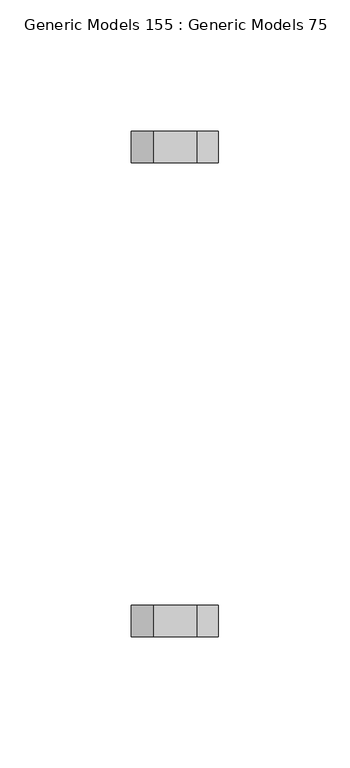
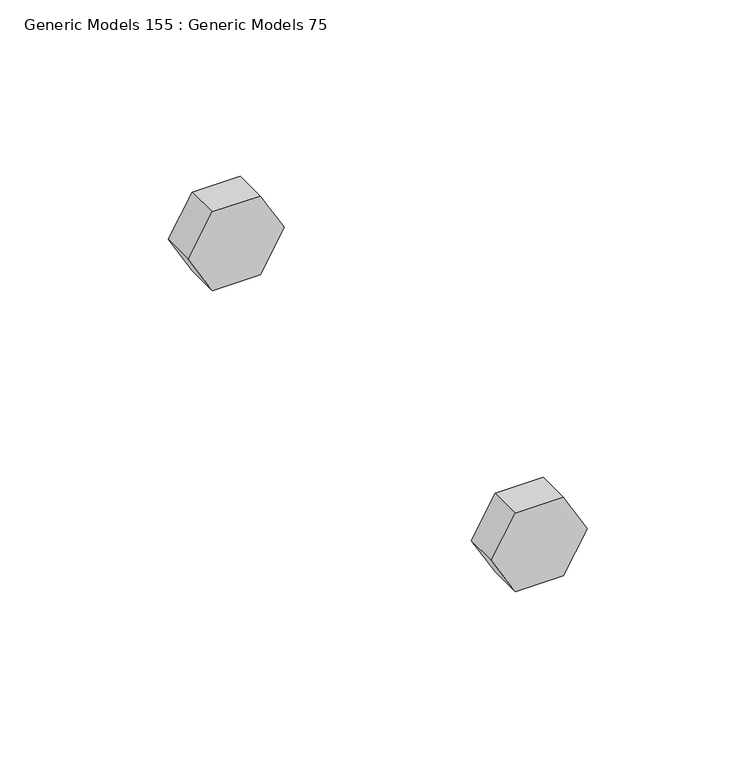
"""IFC4 building model written with IfcOpenShell, lengths in millimetres: proxy geometry, Generic Models 155 : Generic Models 75."""

from ifc_helpers import new_model, si_unit, frame, origin, place, context, project, spatial, polyline, outline, extrude, source, transform, mapped, element, save


def generic_models_155_generic_models_75_12a366e2(model_context):
    return source(origin(), model_context, "Body", "SweptSolid", [
        extrude(outline(polyline([(271657.7625, 31979.8726858), (271657.7625, 31996.3704698), (271672.05, 32004.6193618), (271686.3375, 31996.3704698), (271686.3375, 31979.8726858), (271672.05, 31971.6237939), (271657.7625, 31979.8726858)])), frame((0.0, 36311.3770442, 0.0), z_axis=(0.0, 1.0, 0.0), x_axis=(0.0, 0.0, 1.0)), (0.0, 0.0, 1.0), 11.90625),
        extrude(outline(polyline([(271657.7625, 31979.8726858), (271657.7625, 31996.3704698), (271672.05, 32004.6193618), (271686.3375, 31996.3704698), (271686.3375, 31979.8726858), (271672.05, 31971.6237939), (271657.7625, 31979.8726858)])), frame((0.0, 36491.5582942, 0.0), z_axis=(0.0, 1.0, 0.0), x_axis=(0.0, 0.0, 1.0)), (0.0, 0.0, 1.0), 11.90625),
    ])


if __name__ == "__main__":
    model = new_model("IFC4")
    model_context = context("Model", 3, world=origin())
    ifc_project = project(units=[si_unit("LENGTHUNIT", "METRE", prefix="MILLI")], contexts=[model_context])
    site = spatial("IfcSite", under=ifc_project)
    building = spatial("IfcBuilding", under=site)
    placement = place(None, origin())
    generic_models_155_generic_models_75_shape = generic_models_155_generic_models_75_12a366e2(model_context)
    element("IfcBuildingElementProxy", 1, Name="Generic Models 155 : Generic Models 75", ObjectType="Generic Models 155 : Generic Models 75", at=placement, inside=building, context=model_context, shape_type="MappedRepresentation", body=[
        mapped(generic_models_155_generic_models_75_shape, transform((0.0, 0.0, 0.0), x_axis=(1.0, 0.0, 0.0), y_axis=(0.0, 1.0, 0.0), z_axis=(0.0, 0.0, 1.0))),
    ])
    save(model, "model.ifc")

# Revit data of these elements
# Element 1 (IfcBuildingElementProxy, "Generic Models 155 : Generic Models 75")
#   Materials on its faces: "3/4\" GALV. THRU BOLTS"
# Materials
#   "3/4\" GALV. THRU BOLTS": class "Generic", colour RGB 105 69 171, transparency 0, Cost = 0
